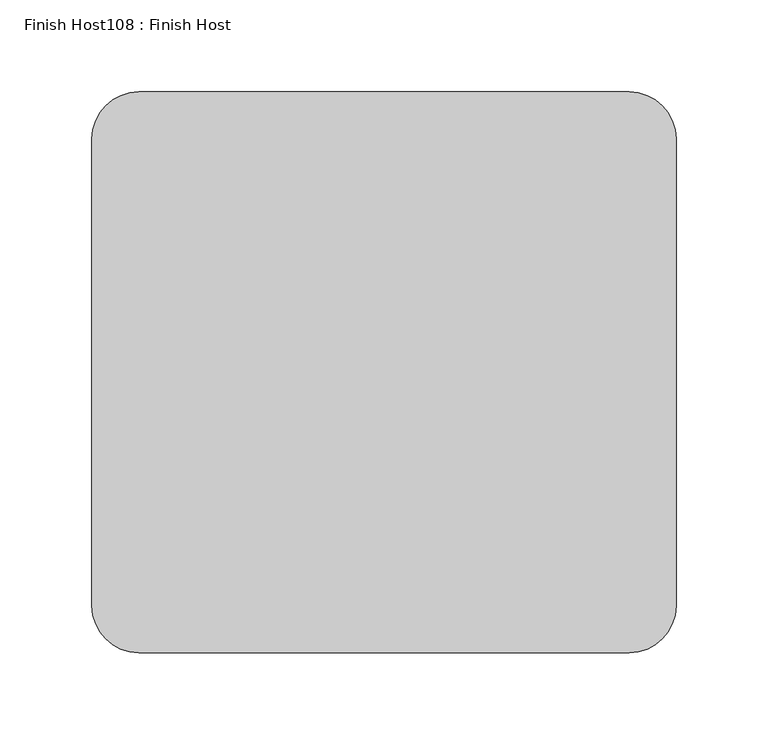
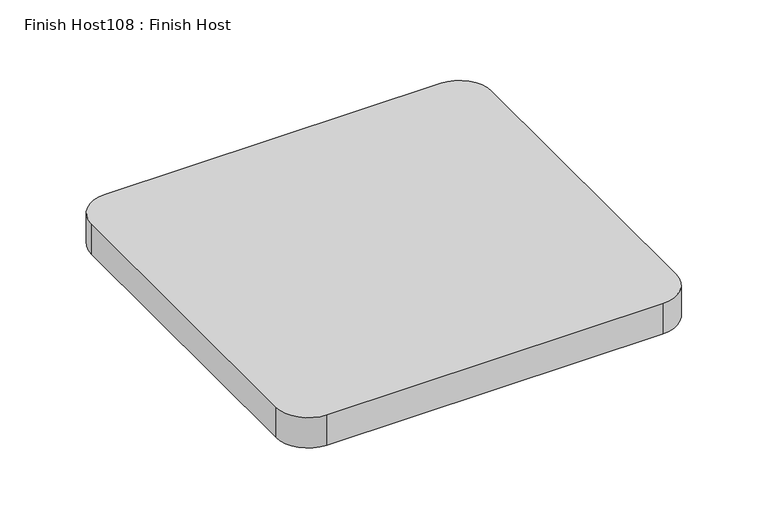
"""IFC4 building model written with IfcOpenShell, lengths in millimetres: proxy geometry, Finish Host108 : Finish Host."""

from ifc_helpers import new_model, si_unit, point, frame_2d, origin, origin_with_axes, place, context, project, spatial, polyline, circle_curve, trimmed, segment, composite_curve, outline, extrude, source, transform, mapped, element, save


def finish_host108_finish_host_dad55fd6(model_context):
    return source(origin(), model_context, "Body", "SweptSolid", [
        extrude(outline(composite_curve([segment(polyline([(701.4157184, 4229.4760864), (701.4157184, 4483.4760864)]), True, "CONTINUOUS"), segment(trimmed(circle_curve(frame_2d((726.8157184, 4483.4760864)), 25.4), [point((701.4157184, 4483.4760864))], [point((726.8157184, 4508.8760864))], False, "CARTESIAN"), True, "CONTINUOUS"), segment(polyline([(726.8157184, 4508.8760864), (993.5157184, 4508.8760864)]), True, "CONTINUOUS"), segment(trimmed(circle_curve(frame_2d((993.5157184, 4483.4760864)), 25.4), [point((993.5157184, 4508.8760864))], [point((1018.9157184, 4483.4760864))], False, "CARTESIAN"), True, "CONTINUOUS"), segment(polyline([(1018.9157184, 4483.4760864), (1018.9157184, 4229.4760864)]), True, "CONTINUOUS"), segment(trimmed(circle_curve(frame_2d((993.5157184, 4229.4760864)), 25.4), [point((1018.9157184, 4229.4760864))], [point((993.5157184, 4204.0760864))], False, "CARTESIAN"), True, "CONTINUOUS"), segment(polyline([(993.5157184, 4204.0760864), (726.8157184, 4204.0760864)]), True, "CONTINUOUS"), segment(trimmed(circle_curve(frame_2d((726.8157184, 4229.4760864)), 25.4), [point((726.8157184, 4204.0760864))], [point((701.4157184, 4229.4760864))], False, "CARTESIAN"), True, "CONTINUOUS")], self_intersect=False)), origin_with_axes(), (0.0, 0.0, 1.0), 25.4),
    ])


if __name__ == "__main__":
    model = new_model("IFC4")
    model_context = context("Model", 3, world=origin())
    ifc_project = project(units=[si_unit("LENGTHUNIT", "METRE", prefix="MILLI")], contexts=[model_context])
    site = spatial("IfcSite", under=ifc_project)
    building = spatial("IfcBuilding", under=site)
    placement = place(None, origin())
    finish_host108_finish_host_shape = finish_host108_finish_host_dad55fd6(model_context)
    element("IfcBuildingElementProxy", 1, Name="Finish Host108 : Finish Host", ObjectType="Finish Host108 : Finish Host", at=placement, inside=building, context=model_context, shape_type="MappedRepresentation", body=[
        mapped(finish_host108_finish_host_shape, transform((0.0, 0.0, 0.0), x_axis=(1.0, 0.0, 0.0), y_axis=(0.0, 1.0, 0.0), z_axis=(0.0, 0.0, 1.0))),
    ])
    save(model, "model.ifc")

# Revit data of these elements
# Type "Finish Host108 : Finish Host"
#   Countertop Material = Fabric - Teknion - T102 - Topology - Natural
# Element 1 (IfcBuildingElementProxy, "Finish Host108 : Finish Host")
#   Materials on its faces: "Fabric - Teknion - T102 - Topology - Natural"
# Materials
#   "Fabric - Teknion - T102 - Topology - Natural": class "Fabric", colour RGB 65 62 55, transparency 0, Model = "T102", Manufacturer = "Teknion Studio", URL = "http://www.teknionstudio.com/", Description = "Natural Topology", Cost = 0
